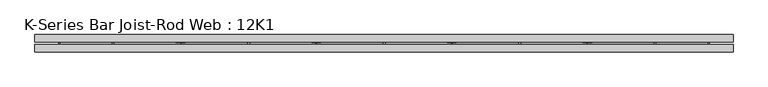
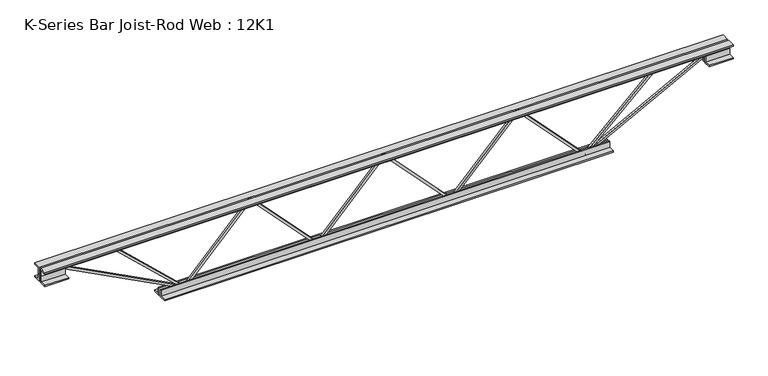
"""IFC4 building model written with IfcOpenShell, lengths in millimetres: beam geometry, K-Series Bar Joist-Rod Web : 12K1."""

from ifc_helpers import new_model, si_unit, frame, origin, place, context, project, spatial, polyline, outline, extrude, source, transform, mapped, element, save


def k_series_bar_joist_rod_web_12k1_28415eb9(model_context):
    return source(origin(), model_context, "Body", "SweptSolid", [
        extrude(outline(polyline([(-141.2875, -283.6333333), (-150.8125, -283.6333333), (-150.8125, -278.4126631), (141.2875, -1.1293297), (141.2875, 1.1293297), (-150.8125, 278.4126631), (-150.8125, 283.6333333), (-141.2875, 283.6333333), (-141.2875, 282.5040036), (150.8125, 5.2206703), (150.8125, -5.2206703), (-141.2875, -282.5040036), (-141.2875, -283.6333333)])), frame((0.0, -4.7625, 0.0), z_axis=(0.0, 1.0, 0.0), x_axis=(0.0, 0.0, 1.0)), (0.0, 0.0, 1.0), 9.525),
        extrude(outline(polyline([(-141.2875, 283.6333333), (-150.8125, 283.6333333), (-150.8125, 288.8540036), (141.2875, 566.1373369), (141.2875, 568.3959964), (-150.8125, 845.6793297), (-150.8125, 850.9), (-141.2875, 850.9), (-141.2875, 849.7706703), (150.8125, 572.4873369), (150.8125, 562.0459964), (-141.2875, 284.7626631), (-141.2875, 283.6333333)])), frame((0.0, -4.7625, 0.0), z_axis=(0.0, 1.0, 0.0), x_axis=(0.0, 0.0, 1.0)), (0.0, 0.0, 1.0), 9.525),
        extrude(outline(polyline([(-141.2875, -850.9), (-150.8125, -850.9), (-150.8125, -845.6793297), (141.2875, -568.3959964), (141.2875, -566.1373369), (-150.8125, -288.8540036), (-150.8125, -283.6333333), (-141.2875, -283.6333333), (-141.2875, -284.7626631), (150.8125, -562.0459964), (150.8125, -572.4873369), (-141.2875, -849.7706703), (-141.2875, -850.9)])), frame((0.0, -4.7625, 0.0), z_axis=(0.0, 1.0, 0.0), x_axis=(0.0, 0.0, 1.0)), (0.0, 0.0, 1.0), 9.525),
        extrude(outline(polyline([(4.7625, 152.4), (36.5125, 152.4), (36.5125, 146.05), (11.1125, 146.05), (11.1125, 120.65), (4.7625, 120.65), (4.7625, 152.4)])), frame((-1460.5, 0.0, 0.0), z_axis=(1.0, 0.0, 0.0), x_axis=(0.0, 1.0, 0.0)), (0.0, 0.0, 1.0), 2921.0),
        extrude(outline(polyline([(-4.7625, 152.4), (-4.7625, 120.65), (-11.1125, 120.65), (-11.1125, 146.05), (-36.5125, 146.05), (-36.5125, 152.4), (-4.7625, 152.4)])), frame((-1460.5, 0.0, 0.0), z_axis=(1.0, 0.0, 0.0), x_axis=(0.0, 1.0, 0.0)), (0.0, 0.0, 1.0), 2921.0),
        extrude(outline(polyline([(-4.7625, 88.9), (-36.5125, 88.9), (-36.5125, 95.25), (-11.1125, 95.25), (-11.1125, 120.65), (-4.7625, 120.65), (-4.7625, 88.9)])), frame((-1460.5, 0.0, 0.0), z_axis=(1.0, 0.0, 0.0), x_axis=(0.0, 1.0, 0.0)), (0.0, 0.0, 1.0), 101.6),
        extrude(outline(polyline([(36.5125, 88.9), (4.7625, 88.9), (4.7625, 120.65), (11.1125, 120.65), (11.1125, 95.25), (36.5125, 95.25), (36.5125, 88.9)])), frame((-1460.5, 0.0, 0.0), z_axis=(1.0, 0.0, 0.0), x_axis=(0.0, 1.0, 0.0)), (0.0, 0.0, 1.0), 101.6),
        extrude(outline(polyline([(4.7625, 88.9), (4.7625, 120.65), (11.1125, 120.65), (11.1125, 95.25), (36.5125, 95.25), (36.5125, 88.9), (4.7625, 88.9)])), frame((1358.9, 0.0, 0.0), z_axis=(1.0, 0.0, 0.0), x_axis=(0.0, 1.0, 0.0)), (0.0, 0.0, 1.0), 101.6),
        extrude(outline(polyline([(-4.7625, 88.9), (-36.5125, 88.9), (-36.5125, 95.25), (-11.1125, 95.25), (-11.1125, 120.65), (-4.7625, 120.65), (-4.7625, 88.9)])), frame((1358.9, 0.0, 0.0), z_axis=(1.0, 0.0, 0.0), x_axis=(0.0, 1.0, 0.0)), (0.0, 0.0, 1.0), 101.6),
        extrude(outline(polyline([(4.7625, -152.4), (4.7625, -120.65), (11.1125, -120.65), (11.1125, -146.05), (36.5125, -146.05), (36.5125, -152.4), (4.7625, -152.4)])), frame((-952.5, 0.0, 0.0), z_axis=(1.0, 0.0, 0.0), x_axis=(0.0, 1.0, 0.0)), (0.0, 0.0, 1.0), 1905.0),
        extrude(outline(polyline([(-4.7625, -152.4), (-36.5125, -152.4), (-36.5125, -146.05), (-11.1125, -146.05), (-11.1125, -120.65), (-4.7625, -120.65), (-4.7625, -152.4)])), frame((-952.5, 0.0, 0.0), z_axis=(1.0, 0.0, 0.0), x_axis=(0.0, 1.0, 0.0)), (0.0, 0.0, 1.0), 1905.0),
        extrude(outline(polyline([(0.0, -9.525), (0.0, 0.0), (573.7533355, 0.0), (573.7533355, -9.525), (0.0, -9.525)])), frame((-1361.1137714, 4.7625, 116.4332925), z_axis=(0.46483389898951394, 0.0, 0.8853979028381569), x_axis=(0.8853979028381569, 0.0, -0.46483389898951394)), (0.0, 0.0, 1.0), 9.525),
        extrude(outline(polyline([(0.0, -9.525), (0.0, 0.0), (389.3285988, 0.0), (389.3285988, -9.525), (0.0, -9.525)])), frame((-1137.7957671, 4.7625, 117.1804276), z_axis=(0.6850254537677595, 0.0, 0.7285191333728136), x_axis=(0.7285191333728136, 0.0, -0.6850254537677595)), (0.0, 0.0, 1.0), 9.525),
        extrude(outline(polyline([(0.0, -9.525), (0.0, 0.0), (573.7533355, 0.0), (573.7533355, -9.525), (0.0, -9.525)])), frame((1361.1137714, -4.7625, 116.4332925), z_axis=(-0.4648338989894941, 0.0, 0.8853979028381673), x_axis=(-0.8853979028381673, 0.0, -0.4648338989894941)), (0.0, 0.0, 1.0), 9.525),
        extrude(outline(polyline([(0.0, -9.525), (0.0, 0.0), (389.3285988, 0.0), (389.3285988, -9.525), (0.0, -9.525)])), frame((1137.7957671, -4.7625, 117.1804276), z_axis=(-0.6850254537677518, 0.0, 0.7285191333728207), x_axis=(-0.7285191333728207, 0.0, -0.6850254537677518)), (0.0, 0.0, 1.0), 9.525),
    ])


if __name__ == "__main__":
    model = new_model("IFC4")
    model_context = context("Model", 3, world=origin())
    ifc_project = project(units=[si_unit("LENGTHUNIT", "METRE", prefix="MILLI")], contexts=[model_context])
    site = spatial("IfcSite", under=ifc_project)
    building = spatial("IfcBuilding", under=site)
    placement = place(None, origin())
    k_series_bar_joist_rod_web_12k1_shape = k_series_bar_joist_rod_web_12k1_28415eb9(model_context)
    element("IfcBeam", 1, ObjectType="K-Series Bar Joist-Rod Web : 12K1", at=placement, inside=building, context=model_context, shape_type="MappedRepresentation", body=[
        mapped(k_series_bar_joist_rod_web_12k1_shape, transform((0.0, 0.0, 0.0), x_axis=(1.0, 0.0, 0.0), y_axis=(0.0, 1.0, 0.0), z_axis=(0.0, 0.0, 1.0))),
    ])
    save(model, "model.ifc")

# Revit data of these elements
# Type "K-Series Bar Joist-Rod Web : 12K1"
#   Assembly Code = "B1010350"
#   Wt = 5
#   Web Thickness = 0' - 0 3/8"
#   Start Offset [instance default] = 0' - 0"
#   Start Extension [instance default] = 0' - 0"
#   Seat Length = 0' - 4"
#   Seat Depth = 0' - 2 1/2"
#   PanelArrayLength [instance default] = 20' - 0"
#   Panel [instance default] = 2' - 0"
#   End Offset [instance default] = 0' - 0"
#   End Extension [instance default] = 0' - 0"
#   End Panel = 2' - 0"
#   Cord Leg = 0' - 1 1/4"
#   Chord Thickness = 0' - 0 1/4"
#   Length [instance default] = 24' - 0"
#   Depth = 1' - 0"
#   PanelArrayNum [instance default] = 10
#   Structural Material = none
# Element 1 (IfcBeam, "K-Series Bar Joist-Rod Web : 12K1")
#   PanelArrayLength = 5' - 7"
#   Panel = 1' - 10.33333"
#   PanelArrayNum = 3
